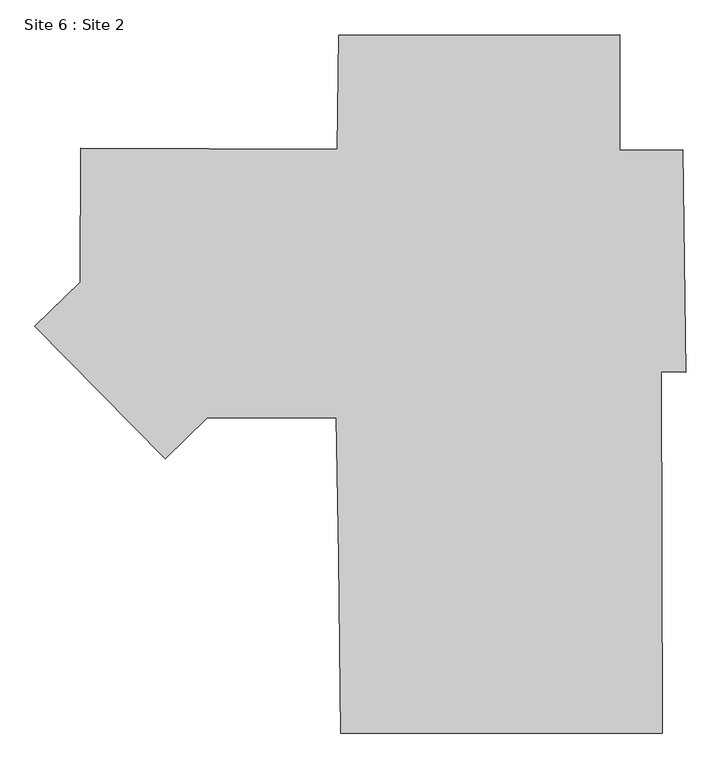
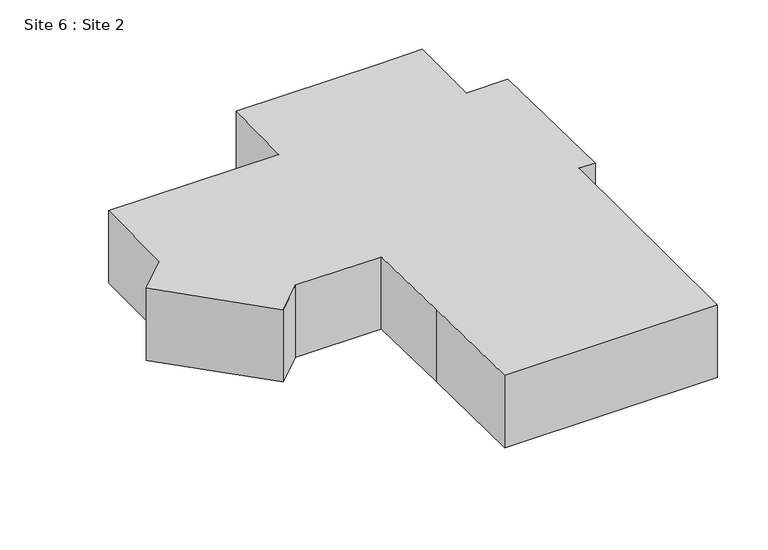
"""IFC4 building model written with IfcOpenShell, lengths in millimetres: geographic element geometry, Site 6 : Site 2."""

from ifc_helpers import new_model, si_unit, frame, origin, place, context, project, spatial, polyline, outline, extrude, source, transform, mapped, element, save


def site_6_site_2_d98898f6(model_context):
    return source(origin(), model_context, "Body", "SweptSolid", [
        extrude(outline(polyline([(-15214.7871008, 111231.0905537), (-11048.1543414, 111272.3359659), (-10855.197666, 96536.2310929), (-12480.6255393, 96559.7790667), (-12420.1240701, 72680.7905545), (-33656.7098652, 72683.6248607), (-33793.7026636, 84269.05712), (-33964.5413496, 93517.9430993), (-42499.5178675, 93539.9829585), (-45282.1665111, 90836.8254736), (-53893.7525646, 99598.386294), (-50904.9826146, 102501.7322056), (-50878.53392, 111341.3262468), (-33910.1680098, 111298.718246), (-33801.2602868, 118816.2078743), (-19575.8102621, 118813.3371712), (-15205.9990186, 118851.6390867), (-15214.7871008, 111231.0905537)])), frame((0.0, 0.0, 266395.2), z_axis=(0.0, 0.0, 1.0), x_axis=(1.0, 0.0, 0.0)), (0.0, 0.0, 1.0), 7620.0),
    ])


if __name__ == "__main__":
    model = new_model("IFC4")
    model_context = context("Model", 3, world=origin())
    ifc_project = project(units=[si_unit("LENGTHUNIT", "METRE", prefix="MILLI")], contexts=[model_context])
    site = spatial("IfcSite", under=ifc_project)
    building = spatial("IfcBuilding", under=site)
    placement = place(None, origin())
    site_6_site_2_shape = site_6_site_2_d98898f6(model_context)
    element("IfcGeographicElement", 1, ObjectType="Site 6 : Site 2", at=placement, inside=building, context=model_context, shape_type="MappedRepresentation", body=[
        mapped(site_6_site_2_shape, transform((0.0, 0.0, 0.0), x_axis=(1.0, 0.0, 0.0), y_axis=(0.0, 1.0, 0.0), z_axis=(0.0, 0.0, 1.0))),
    ])
    save(model, "model.ifc")

# Revit data of these elements
# Element 1 (IfcGeographicElement, "Site 6 : Site 2")
#   Materials on its faces: "EXISTING BUILDING"
# Materials
#   "EXISTING BUILDING": class "Generic", colour RGB 120 120 120, transparency 0, Cost = 0
